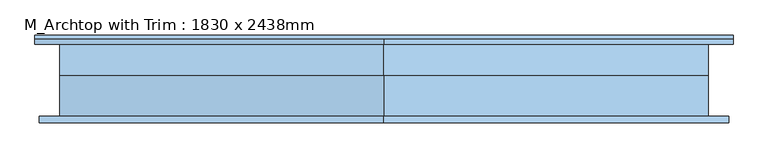
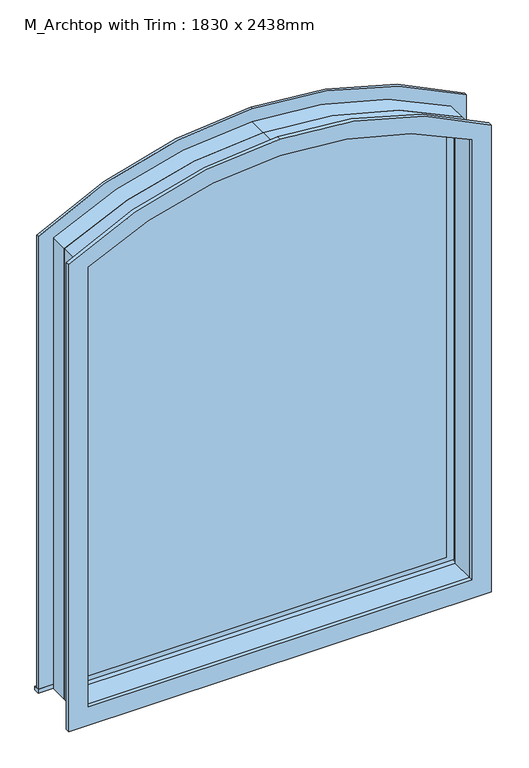
"""IFC4 building model written with IfcOpenShell, lengths in millimetres: window geometry, M_Archtop with Trim : 1830 x 2438mm."""

import ifcopenshell
import ifcopenshell.guid

model = None  # the IFC model being written
_history = None  # IfcOwnerHistory: only IFC2X3 demands one
_inside = {}  # id of a spatial element -> (the spatial element, [elements in it])
_under = {}  # id of a project, library or spatial element -> (it, [spatial elements below it])
_declared = {}  # id of a project -> (the project, [libraries it declares])
_typed = {}  # id of a type object -> (the type object, [elements of that type])
_made_of = {}  # id of a material, layer set ... -> (it, [elements and type objects made of it])


def new_model(schema):
    """Start an empty IFC model of exactly this schema.

    Asked for "IFC4X3", IfcOpenShell would pick the latest addendum, in which some entities
    have other attributes; the version numbers below select the first issue.
    IFC2X3 requires an IfcOwnerHistory on every rooted entity: one is made here for all.
    """
    global model, _history
    if schema == "IFC4X3":
        model = ifcopenshell.file(schema_version=(4, 3, 0, 0))
    else:
        model = ifcopenshell.file(schema=schema)
    _inside.clear()
    _under.clear()
    _declared.clear()
    _typed.clear()
    _made_of.clear()
    _history = None
    if model.schema == "IFC2X3":
        org = make("IfcOrganization", Name="unknown")
        user = make(
            "IfcPersonAndOrganization",
            ThePerson=make("IfcPerson", FamilyName="unknown"),
            TheOrganization=org,
        )
        app = make(
            "IfcApplication",
            ApplicationDeveloper=org,
            Version="unknown",
            ApplicationFullName="unknown",
            ApplicationIdentifier="unknown",
        )
        _history = make(
            "IfcOwnerHistory",
            OwningUser=user,
            OwningApplication=app,
            ChangeAction="ADDED",
            CreationDate=0,
        )
    return model


def make(cls, **values):
    """One entity of the class cls with the attributes given. An attribute that is None is left unset."""
    return model.create_entity(
        cls, **{name: value for name, value in values.items() if value is not None}
    )


def rooted(cls, **values):
    """An entity with a GlobalId (a new one), such as an element, a storey or a relation."""
    return make(cls, GlobalId=ifcopenshell.guid.new(), OwnerHistory=_history, **values)


def si_unit(unit_type, name, prefix=None):
    """IfcSIUnit, for example si_unit("LENGTHUNIT", "METRE", prefix="MILLI")."""
    return make("IfcSIUnit", UnitType=unit_type, Prefix=prefix, Name=name)


def assignment(units):
    """IfcUnitAssignment: the units of a project."""
    return None if units is None else make("IfcUnitAssignment", Units=units)


def point(xyz):
    """IfcCartesianPoint."""
    return None if xyz is None else make("IfcCartesianPoint", Coordinates=xyz)


def direction(xyz):
    """IfcDirection."""
    return None if xyz is None else make("IfcDirection", DirectionRatios=xyz)


def frame(location, z_axis=None, x_axis=None):
    """IfcAxis2Placement3D, a coordinate frame: its origin and axes. An axis left out is left unset."""
    return make(
        "IfcAxis2Placement3D",
        Location=point(location),
        Axis=direction(z_axis),
        RefDirection=direction(x_axis),
    )


def frame_2d(location, x_axis=None):
    """IfcAxis2Placement2D, a coordinate frame in the plane: its origin and x axis."""
    return make(
        "IfcAxis2Placement2D", Location=point(location), RefDirection=direction(x_axis)
    )


def origin():
    """The frame at (0, 0, 0) with its axes left unset."""
    return frame((0.0, 0.0, 0.0))


def place(relative_to, where):
    """IfcLocalPlacement: puts the frame where relative to a parent placement (None: the world)."""
    return make(
        "IfcLocalPlacement", PlacementRelTo=relative_to, RelativePlacement=where
    )


def context(
    kind, dimensions, precision=None, world=None, true_north=None, identifier=None
):
    """IfcGeometricRepresentationContext, for example the 3D "Model" context."""
    return make(
        "IfcGeometricRepresentationContext",
        ContextIdentifier=identifier,
        ContextType=kind,
        CoordinateSpaceDimension=dimensions,
        Precision=precision,
        WorldCoordinateSystem=world,
        TrueNorth=true_north,
    )


def project(units=None, contexts=None):
    """IfcProject with its units and contexts."""
    return rooted(
        "IfcProject",
        Name="project",
        RepresentationContexts=contexts,
        UnitsInContext=assignment(units),
    )


def spatial(cls, under=None, at=None, **own):
    """A site, building, storey or space (cls), placed at a placement, below another one or the project."""
    s = rooted(cls, ObjectPlacement=at, **own)
    if under is not None:
        _under.setdefault(under.id(), (under, []))[1].append(s)
    return s


def polyline(points):
    """IfcPolyline through the points."""
    return make("IfcPolyline", Points=[point(p) for p in points])


def circle_curve(where, radius):
    """IfcCircle in the frame where."""
    return make("IfcCircle", Position=where, Radius=radius)


def trimmed(basis, trim1, trim2, sense, master):
    """IfcTrimmedCurve: the piece of a basis curve between two trims."""
    return make(
        "IfcTrimmedCurve",
        BasisCurve=basis,
        Trim1=trim1,
        Trim2=trim2,
        SenseAgreement=sense,
        MasterRepresentation=master,
    )


def segment(curve, same_sense, transition):
    """IfcCompositeCurveSegment."""
    return make(
        "IfcCompositeCurveSegment",
        Transition=transition,
        SameSense=same_sense,
        ParentCurve=curve,
    )


def composite_curve(segments, self_intersect=None):
    """IfcCompositeCurve: segments joined end to end."""
    return make("IfcCompositeCurve", Segments=segments, SelfIntersect=self_intersect)


def outline(outer, holes=None, kind="AREA"):
    """IfcArbitraryClosedProfileDef: a profile drawn as a closed curve; with holes, ...WithVoids."""
    if holes is None:
        return make("IfcArbitraryClosedProfileDef", ProfileType=kind, OuterCurve=outer)
    return make(
        "IfcArbitraryProfileDefWithVoids",
        ProfileType=kind,
        OuterCurve=outer,
        InnerCurves=holes,
    )


def extrude(swept, where, along, depth):
    """IfcExtrudedAreaSolid: the profile swept, set in the frame where, extruded along a direction by depth."""
    return make(
        "IfcExtrudedAreaSolid",
        SweptArea=swept,
        Position=where,
        ExtrudedDirection=direction(along),
        Depth=depth,
    )


def shape(context_of_items, identifier, shape_type, items):
    """IfcShapeRepresentation: the items that make up one representation, for example the "Body"."""
    return make(
        "IfcShapeRepresentation",
        ContextOfItems=context_of_items,
        RepresentationIdentifier=identifier,
        RepresentationType=shape_type,
        Items=items,
    )


def source(mapping_origin, context_of_items, identifier, shape_type, items):
    """IfcRepresentationMap: a shape defined once, which mapped items show again and again."""
    return make(
        "IfcRepresentationMap",
        MappingOrigin=mapping_origin,
        MappedRepresentation=shape(context_of_items, identifier, shape_type, items),
    )


def transform(
    local_origin,
    x_axis=None,
    y_axis=None,
    z_axis=None,
    scale=None,
    scale2=None,
    scale3=None,
    uniform=True,
):
    """IfcCartesianTransformationOperator3D, or its non-uniform kind. x_axis, y_axis, z_axis: its Axis1, 2, 3."""
    if uniform:
        return make(
            "IfcCartesianTransformationOperator3D",
            Axis1=direction(x_axis),
            Axis2=direction(y_axis),
            LocalOrigin=point(local_origin),
            Scale=scale,
            Axis3=direction(z_axis),
        )
    return make(
        "IfcCartesianTransformationOperator3DnonUniform",
        Axis1=direction(x_axis),
        Axis2=direction(y_axis),
        LocalOrigin=point(local_origin),
        Scale=scale,
        Axis3=direction(z_axis),
        Scale2=scale2,
        Scale3=scale3,
    )


def mapped(mapping_source, mapping_target):
    """IfcMappedItem: shows the shape of a source again, moved by a transform."""
    return make(
        "IfcMappedItem", MappingSource=mapping_source, MappingTarget=mapping_target
    )


def made_of(thing, what):
    """Note that an element or type object is made of a material, layer set ...; save() writes the relation."""
    if what is not None:
        _made_of.setdefault(what.id(), (what, []))[1].append(thing)
    return thing


def element(
    cls,
    number,
    at=None,
    inside=None,
    cuts=None,
    type_object=None,
    material=None,
    context=None,
    identifier="Body",
    shape_type=None,
    held_by="IfcProductDefinitionShape",
    body=None,
    shapes=None,
    **own,
):
    """One element of the class cls, such as IfcWall. Its Tag is "e" and its number.

    at: its placement. inside: the storey or other place that contains it. cuts: it is an
    opening in that element (IfcRelVoidsElement). A single representation is given by context,
    identifier, shape_type and body (its items); several are given by shapes. held_by: the class
    of the entity that holds the representations. save() writes the other relations.
    """
    e = rooted(cls, Tag="e%d" % number, ObjectPlacement=at, **own)
    if body is not None:
        shapes = [shape(context, identifier, shape_type, body)]
    if shapes is not None:
        e.Representation = make(held_by, Representations=shapes)
    if inside is not None:
        _inside.setdefault(inside.id(), (inside, []))[1].append(e)
    if cuts is not None:
        rooted(
            "IfcRelVoidsElement", RelatingBuildingElement=cuts, RelatedOpeningElement=e
        )
    if type_object is not None:
        _typed.setdefault(type_object.id(), (type_object, []))[1].append(e)
    return made_of(e, material)


def aggregate(whole, parts):
    """IfcRelAggregates: a whole, such as a stair, and the parts it consists of."""
    return rooted("IfcRelAggregates", RelatingObject=whole, RelatedObjects=parts)


def save(model, path):
    """Write the relations noted so far, then the file.

    IfcRelAggregates (storeys below a building ...), IfcRelContainedInSpatialStructure (elements
    in a storey), IfcRelDefinesByType, IfcRelAssociatesMaterial and IfcRelDeclares: one each for
    every whole, place, type object, material and project.
    """
    for whole, parts in _under.values():
        aggregate(whole, parts)
    for where, things in _inside.values():
        rooted(
            "IfcRelContainedInSpatialStructure",
            RelatedElements=things,
            RelatingStructure=where,
        )
    for kind, things in _typed.values():
        rooted("IfcRelDefinesByType", RelatedObjects=things, RelatingType=kind)
    for what, things in _made_of.values():
        rooted("IfcRelAssociatesMaterial", RelatedObjects=things, RelatingMaterial=what)
    for by, libraries in _declared.values():
        rooted("IfcRelDeclares", RelatingContext=by, RelatedDefinitions=libraries)
    model.write(path)


def m_archtop_with_trim_1830_x_2438mm_7157e706(model_context):
    return source(origin(), model_context, "Body", "SweptSolid", [
        extrude(outline(composite_curve([segment(polyline([(336.75, 903.8802979), (2486.7895349, 903.8802979)]), True, "CONTINUOUS"), segment(trimmed(circle_curve(frame_2d((913.0, 7.9302979)), 1810.95), [point((2486.7895349, 903.8802979))], [point((2723.95, 7.9302979))], False, "CARTESIAN"), True, "CONTINUOUS"), segment(trimmed(circle_curve(frame_2d((913.0, 7.9302979)), 1810.95), [point((2723.95, 7.9302979))], [point((2486.7895349, -888.019702))], False, "CARTESIAN"), True, "CONTINUOUS"), segment(polyline([(2486.7895349, -888.019702), (336.75, -888.019702), (336.75, 903.8802979)]), True, "CONTINUOUS")], self_intersect=False), holes=[composite_curve([segment(polyline([(368.5, 859.4302979), (368.5, -843.5697021), (2464.3533948, -843.5697021)]), True, "CONTINUOUS"), segment(trimmed(circle_curve(frame_2d((913.0, 7.9302979)), 1769.675), [point((2464.3533948, -843.5697021))], [point((2682.675, 7.9302979))], True, "CARTESIAN"), True, "CONTINUOUS"), segment(trimmed(circle_curve(frame_2d((913.0, 7.9302979)), 1769.675), [point((2682.675, 7.9302979))], [point((2464.3533948, 859.4302979))], True, "CARTESIAN"), True, "CONTINUOUS"), segment(polyline([(2464.3533948, 859.4302979), (368.5, 859.4302979)]), True, "CONTINUOUS")], self_intersect=False)]), frame((0.0, 38.1, 0.0), z_axis=(0.0, 1.0, 0.0), x_axis=(0.0, 0.0, 1.0)), (0.0, 0.0, 1.0), 44.45),
        extrude(outline(polyline([(-972.9697019, 127.3), (996.930298, 127.3), (996.930298, 101.6), (-972.9697019, 101.6), (-972.9697019, 127.3)])), frame((0.0, 0.0, 305.0), z_axis=(0.0, 0.0, 1.0), x_axis=(1.0, 0.0, 0.0)), (0.0, 0.0, 1.0), 19.05),
        extrude(outline(composite_curve([segment(polyline([(324.05, 907.9302979), (324.05, 996.930298), (2527.9180866, 996.930298)]), True, "CONTINUOUS"), segment(trimmed(circle_curve(frame_2d((913.0, 11.980298)), 1891.5831805), [point((2527.9180866, 996.930298))], [point((2804.5831805, 11.980298))], False, "CARTESIAN"), True, "CONTINUOUS"), segment(trimmed(circle_curve(frame_2d((913.0, 11.980298)), 1891.5831805), [point((2804.5831805, 11.980298))], [point((2527.9180866, -972.9697019))], False, "CARTESIAN"), True, "CONTINUOUS"), segment(polyline([(2527.9180866, -972.9697019), (324.05, -972.9697019), (324.05, -883.969702), (2486.7895348, -883.969702)]), True, "CONTINUOUS"), segment(trimmed(circle_curve(frame_2d((913.0, 11.980298)), 1810.95), [point((2486.7895348, -883.969702))], [point((2723.95, 11.980298))], True, "CARTESIAN"), True, "CONTINUOUS"), segment(trimmed(circle_curve(frame_2d((913.0, 11.980298)), 1810.95), [point((2723.95, 11.980298))], [point((2486.7895349, 907.9302979))], True, "CARTESIAN"), True, "CONTINUOUS"), segment(polyline([(2486.7895349, 907.9302979), (324.05, 907.9302979)]), True, "CONTINUOUS")], self_intersect=False)), frame((0.0, 101.6, 0.0), z_axis=(0.0, 1.0, 0.0), x_axis=(0.0, 0.0, 1.0)), (0.0, 0.0, 1.0), 13.0),
        extrude(outline(composite_curve([segment(polyline([(247.75, -960.269702), (247.75, 984.2302979), (2520.8214166, 984.2302979)]), True, "CONTINUOUS"), segment(trimmed(circle_curve(frame_2d((913.0, 11.980298)), 1878.9251635), [point((2520.8214166, 984.2302979))], [point((2791.9251635, 11.980298))], False, "CARTESIAN"), True, "CONTINUOUS"), segment(trimmed(circle_curve(frame_2d((913.0, 11.980298)), 1878.9251635), [point((2791.9251635, 11.980298))], [point((2520.8214165, -960.269702))], False, "CARTESIAN"), True, "CONTINUOUS"), segment(polyline([(2520.8214165, -960.269702), (247.75, -960.269702)]), True, "CONTINUOUS")], self_intersect=False), holes=[composite_curve([segment(polyline([(336.75, -871.2697029), (2479.3883613, -871.2697029)]), True, "CONTINUOUS"), segment(trimmed(circle_curve(frame_2d((913.0, 11.980298)), 1798.25), [point((2479.3883613, -871.2697029))], [point((2711.25, 11.980298))], True, "CARTESIAN"), True, "CONTINUOUS"), segment(trimmed(circle_curve(frame_2d((913.0000002, 11.980298)), 1798.2499998), [point((2711.25, 11.980298))], [point((2479.3883613, 895.2302988))], True, "CARTESIAN"), True, "CONTINUOUS"), segment(polyline([(2479.3883613, 895.2302988), (336.75, 895.2302988), (336.75, -871.2697029)]), True, "CONTINUOUS")], self_intersect=False)]), frame((0.0, -120.6, 0.0), z_axis=(0.0, 1.0, 0.0), x_axis=(0.0, 0.0, 1.0)), (0.0, 0.0, 1.0), 19.0),
        extrude(outline(composite_curve([segment(polyline([(368.5, -839.519702), (368.5, 863.4802977), (2464.6545931, 863.4802977)]), True, "CONTINUOUS"), segment(trimmed(circle_curve(frame_2d((913.0, 11.980298)), 1769.9390458), [point((2464.6545931, 863.4802977))], [point((2682.9390458, 11.980298))], False, "CARTESIAN"), True, "CONTINUOUS"), segment(trimmed(circle_curve(frame_2d((913.0, 11.980298)), 1769.9390458), [point((2682.9390458, 11.980298))], [point((2464.6545929, -839.519702))], False, "CARTESIAN"), True, "CONTINUOUS"), segment(polyline([(2464.6545929, -839.519702), (368.5, -839.519702)]), True, "CONTINUOUS")], self_intersect=False)), frame((0.0, 28.575, 0.0), z_axis=(0.0, 1.0, 0.0), x_axis=(0.0, 0.0, 1.0)), (0.0, 0.0, 1.0), 12.7),
        extrude(outline(composite_curve([segment(polyline([(305.0, 926.980298), (2497.8264889, 926.980298)]), True, "CONTINUOUS"), segment(trimmed(circle_curve(frame_2d((913.0, 11.980298)), 1830.0), [point((2497.8264889, 926.980298))], [point((2743.0, 11.980298))], False, "CARTESIAN"), True, "CONTINUOUS"), segment(trimmed(circle_curve(frame_2d((913.0, 11.980298)), 1830.0), [point((2743.0, 11.980298))], [point((2497.8264889, -903.019702))], False, "CARTESIAN"), True, "CONTINUOUS"), segment(polyline([(2497.8264889, -903.019702), (305.0, -903.019702), (305.0, 926.980298)]), True, "CONTINUOUS")], self_intersect=False), holes=[composite_curve([segment(polyline([(336.75, 895.2302988), (336.75, -871.269702), (2482.779909, -871.269702)]), True, "CONTINUOUS"), segment(trimmed(circle_curve(frame_2d((913.0, 11.980298)), 1801.2050203), [point((2482.779909, -871.269702))], [point((2714.2050203, 11.980298))], True, "CARTESIAN"), True, "CONTINUOUS"), segment(trimmed(circle_curve(frame_2d((913.0, 11.980298)), 1801.2050203), [point((2714.2050203, 11.980298))], [point((2482.7799085, 895.2302988))], True, "CARTESIAN"), True, "CONTINUOUS"), segment(polyline([(2482.7799085, 895.2302988), (336.75, 895.2302988)]), True, "CONTINUOUS")], self_intersect=False)]), frame((0.0, -101.6, 0.0), z_axis=(0.0, 1.0, 0.0), x_axis=(0.0, 0.0, 1.0)), (0.0, 0.0, 1.0), 114.3),
        extrude(outline(composite_curve([segment(polyline([(305.0, -903.019702), (305.0, 926.980298), (2497.8264889, 926.980298)]), True, "CONTINUOUS"), segment(trimmed(circle_curve(frame_2d((913.0, 11.980298)), 1830.0), [point((2497.8264889, 926.980298))], [point((2743.0, 11.980298))], False, "CARTESIAN"), True, "CONTINUOUS"), segment(trimmed(circle_curve(frame_2d((913.0, 11.980298)), 1830.0), [point((2743.0, 11.980298))], [point((2497.8264889, -903.019702))], False, "CARTESIAN"), True, "CONTINUOUS"), segment(polyline([(2497.8264889, -903.019702), (305.0, -903.019702)]), True, "CONTINUOUS")], self_intersect=False), holes=[composite_curve([segment(polyline([(324.05, -883.969702), (2488.8332662, -883.969702)]), True, "CONTINUOUS"), segment(trimmed(circle_curve(frame_2d((913.0, 11.980298)), 1812.726368), [point((2488.8332662, -883.969702))], [point((2725.726368, 11.980298))], True, "CARTESIAN"), True, "CONTINUOUS"), segment(trimmed(circle_curve(frame_2d((913.0, 11.980298)), 1812.726368), [point((2725.726368, 11.980298))], [point((2488.8332662, 907.930298))], True, "CARTESIAN"), True, "CONTINUOUS"), segment(polyline([(2488.8332662, 907.930298), (324.05, 907.930298), (324.05, -883.969702)]), True, "CONTINUOUS")], self_intersect=False)]), frame((0.0, 12.7, 0.0), z_axis=(0.0, 1.0, 0.0), x_axis=(0.0, 0.0, 1.0)), (0.0, 0.0, 1.0), 88.9),
    ])


if __name__ == "__main__":
    model = new_model("IFC4")
    model_context = context("Model", 3, world=origin())
    ifc_project = project(units=[si_unit("LENGTHUNIT", "METRE", prefix="MILLI")], contexts=[model_context])
    site = spatial("IfcSite", under=ifc_project)
    building = spatial("IfcBuilding", under=site)
    placement = place(None, origin())
    m_archtop_with_trim_1830_x_2438mm_shape = m_archtop_with_trim_1830_x_2438mm_7157e706(model_context)
    element("IfcWindow", 1, ObjectType="M_Archtop with Trim : 1830 x 2438mm", at=placement, inside=building, context=model_context, shape_type="MappedRepresentation", body=[
        mapped(m_archtop_with_trim_1830_x_2438mm_shape, transform((0.0, 0.0, 0.0), x_axis=(1.0, 0.0, 0.0), y_axis=(0.0, 1.0, 0.0), z_axis=(0.0, 0.0, 1.0))),
    ])
    save(model, "model.ifc")

# Revit data of these elements
# Type "M_Archtop with Trim : 1830 x 2438mm"
#   Type Mark = "16"
#   Construction Type Id = "GSP4R"
#   Analytic Construction = "1/8 in Pilkington single glazing"
#   Visual Light Transmittance = 0.9
#   Solar Heat Gain Coefficient = 0.78
#   Heat Transfer Coefficient (U) = 3.6886 W/(m²·K)
#   Height = 7' - 11.98425"
#   Radius = 6' - 0.04724"
#   Default Sill Height = 1' - 0.00787"
#   Trim Projection - Ext. = 0' - 0.51181"
#   Trim Projection - Int. = 0' - 0.74803"
#   Trim Width - Exterior = 0' - 3.50394"
#   Trim Width - Interior = 0' - 3.50394"
#   Width = 6' - 0.04724"
#   Glass Pane Material = Glass
#   Sash = Sash
#   Trim Exterior Material = Trim
#   Trim Interior Material = Trim
#   Wall Closure = (empty or 0)
# Element 1 (IfcWindow, "M_Archtop with Trim : 1830 x 2438mm")
#   Materials on its faces: "Trim", "Sash", "Glass"
# Materials
#   "Glass": class "Glass", colour RGB 0 128 192, transparency 0.75, Description = "Soda Lime Glass", Cost = 0
#   "Sash": class "Wood", colour RGB 224 178 126, transparency 0, Cost = 0
#   "Trim": class "Wood", colour RGB 224 178 126, transparency 0
